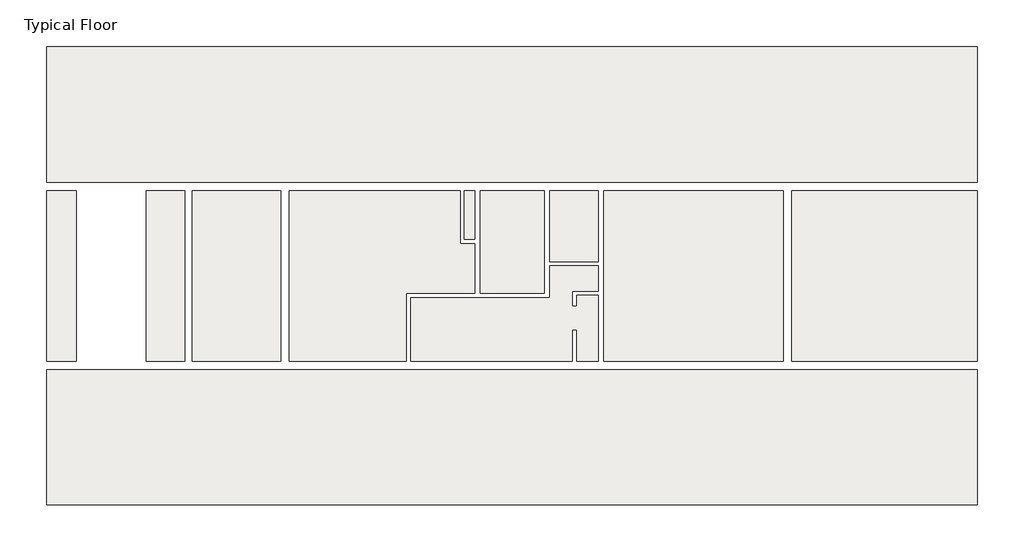
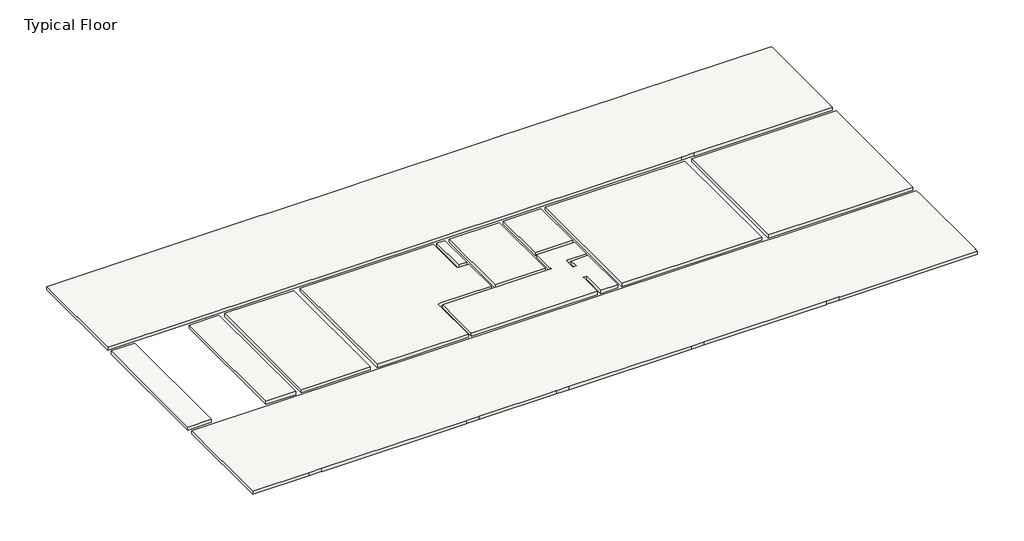
# One storey: 12 slabs.
"""IFC4 building model written with IfcOpenShell, lengths in millimetres."""

import ifcopenshell
import ifcopenshell.guid

model = None  # the IFC model being written
_history = None  # IfcOwnerHistory: only IFC2X3 demands one
_inside = {}  # id of a spatial element -> (the spatial element, [elements in it])
_under = {}  # id of a project, library or spatial element -> (it, [spatial elements below it])
_declared = {}  # id of a project -> (the project, [libraries it declares])
_typed = {}  # id of a type object -> (the type object, [elements of that type])
_made_of = {}  # id of a material, layer set ... -> (it, [elements and type objects made of it])


def new_model(schema):
    """Start an empty IFC model of exactly this schema.

    Asked for "IFC4X3", IfcOpenShell would pick the latest addendum, in which some entities
    have other attributes; the version numbers below select the first issue.
    IFC2X3 requires an IfcOwnerHistory on every rooted entity: one is made here for all.
    """
    global model, _history
    if schema == "IFC4X3":
        model = ifcopenshell.file(schema_version=(4, 3, 0, 0))
    else:
        model = ifcopenshell.file(schema=schema)
    _inside.clear()
    _under.clear()
    _declared.clear()
    _typed.clear()
    _made_of.clear()
    _history = None
    if model.schema == "IFC2X3":
        org = make("IfcOrganization", Name="unknown")
        user = make(
            "IfcPersonAndOrganization",
            ThePerson=make("IfcPerson", FamilyName="unknown"),
            TheOrganization=org,
        )
        app = make(
            "IfcApplication",
            ApplicationDeveloper=org,
            Version="unknown",
            ApplicationFullName="unknown",
            ApplicationIdentifier="unknown",
        )
        _history = make(
            "IfcOwnerHistory",
            OwningUser=user,
            OwningApplication=app,
            ChangeAction="ADDED",
            CreationDate=0,
        )
    return model


def make(cls, **values):
    """One entity of the class cls with the attributes given. An attribute that is None is left unset."""
    return model.create_entity(
        cls, **{name: value for name, value in values.items() if value is not None}
    )


def rooted(cls, **values):
    """An entity with a GlobalId (a new one), such as an element, a storey or a relation."""
    return make(cls, GlobalId=ifcopenshell.guid.new(), OwnerHistory=_history, **values)


def si_unit(unit_type, name, prefix=None):
    """IfcSIUnit, for example si_unit("LENGTHUNIT", "METRE", prefix="MILLI")."""
    return make("IfcSIUnit", UnitType=unit_type, Prefix=prefix, Name=name)


def assignment(units):
    """IfcUnitAssignment: the units of a project."""
    return None if units is None else make("IfcUnitAssignment", Units=units)


def point(xyz):
    """IfcCartesianPoint."""
    return None if xyz is None else make("IfcCartesianPoint", Coordinates=xyz)


def direction(xyz):
    """IfcDirection."""
    return None if xyz is None else make("IfcDirection", DirectionRatios=xyz)


def frame(location, z_axis=None, x_axis=None):
    """IfcAxis2Placement3D, a coordinate frame: its origin and axes. An axis left out is left unset."""
    return make(
        "IfcAxis2Placement3D",
        Location=point(location),
        Axis=direction(z_axis),
        RefDirection=direction(x_axis),
    )


def origin():
    """The frame at (0, 0, 0) with its axes left unset."""
    return frame((0.0, 0.0, 0.0))


def place(relative_to, where):
    """IfcLocalPlacement: puts the frame where relative to a parent placement (None: the world)."""
    return make(
        "IfcLocalPlacement", PlacementRelTo=relative_to, RelativePlacement=where
    )


def context(
    kind, dimensions, precision=None, world=None, true_north=None, identifier=None
):
    """IfcGeometricRepresentationContext, for example the 3D "Model" context."""
    return make(
        "IfcGeometricRepresentationContext",
        ContextIdentifier=identifier,
        ContextType=kind,
        CoordinateSpaceDimension=dimensions,
        Precision=precision,
        WorldCoordinateSystem=world,
        TrueNorth=true_north,
    )


def project(units=None, contexts=None):
    """IfcProject with its units and contexts."""
    return rooted(
        "IfcProject",
        Name="project",
        RepresentationContexts=contexts,
        UnitsInContext=assignment(units),
    )


def spatial(cls, under=None, at=None, **own):
    """A site, building, storey or space (cls), placed at a placement, below another one or the project."""
    s = rooted(cls, ObjectPlacement=at, **own)
    if under is not None:
        _under.setdefault(under.id(), (under, []))[1].append(s)
    return s


def polyline(points):
    """IfcPolyline through the points."""
    return make("IfcPolyline", Points=[point(p) for p in points])


def outline(outer, holes=None, kind="AREA"):
    """IfcArbitraryClosedProfileDef: a profile drawn as a closed curve; with holes, ...WithVoids."""
    if holes is None:
        return make("IfcArbitraryClosedProfileDef", ProfileType=kind, OuterCurve=outer)
    return make(
        "IfcArbitraryProfileDefWithVoids",
        ProfileType=kind,
        OuterCurve=outer,
        InnerCurves=holes,
    )


def extrude(swept, where, along, depth):
    """IfcExtrudedAreaSolid: the profile swept, set in the frame where, extruded along a direction by depth."""
    return make(
        "IfcExtrudedAreaSolid",
        SweptArea=swept,
        Position=where,
        ExtrudedDirection=direction(along),
        Depth=depth,
    )


def faces_of(points, faces, orient=None, outer=None):
    """IfcFace entities. A face is a list of loops; a loop is a list of indices into points, from 0.

    orient and outer hold one flag for each loop. By default every Orientation is true, the
    first loop of a face is its IfcFaceOuterBound and the others are IfcFaceBound.
    """
    made = []
    for i, loops in enumerate(faces):
        bounds = []
        for j, loop in enumerate(loops):
            is_outer = j == 0 if outer is None else outer[i][j]
            bounds.append(
                make(
                    "IfcFaceOuterBound" if is_outer else "IfcFaceBound",
                    Bound=make("IfcPolyLoop", Polygon=[points[k] for k in loop]),
                    Orientation=True if orient is None else orient[i][j],
                )
            )
        made.append(make("IfcFace", Bounds=bounds))
    return made


def faceted_brep(points, faces, orient=None, outer=None, voids=None):
    """IfcFacetedBrep: a solid bounded by flat faces; with voids (closed shells), ...WithVoids."""
    shared = [point(p) for p in points]
    hull = make("IfcClosedShell", CfsFaces=faces_of(shared, faces, orient, outer))
    if voids is None:
        return make("IfcFacetedBrep", Outer=hull)
    return make(
        "IfcFacetedBrepWithVoids",
        Outer=hull,
        Voids=[
            make(cls, CfsFaces=faces_of(shared, fs, o, b)) for cls, fs, o, b in voids
        ],
    )


def shape(context_of_items, identifier, shape_type, items):
    """IfcShapeRepresentation: the items that make up one representation, for example the "Body"."""
    return make(
        "IfcShapeRepresentation",
        ContextOfItems=context_of_items,
        RepresentationIdentifier=identifier,
        RepresentationType=shape_type,
        Items=items,
    )


def made_of(thing, what):
    """Note that an element or type object is made of a material, layer set ...; save() writes the relation."""
    if what is not None:
        _made_of.setdefault(what.id(), (what, []))[1].append(thing)
    return thing


def element(
    cls,
    number,
    at=None,
    inside=None,
    cuts=None,
    type_object=None,
    material=None,
    context=None,
    identifier="Body",
    shape_type=None,
    held_by="IfcProductDefinitionShape",
    body=None,
    shapes=None,
    **own,
):
    """One element of the class cls, such as IfcWall. Its Tag is "e" and its number.

    at: its placement. inside: the storey or other place that contains it. cuts: it is an
    opening in that element (IfcRelVoidsElement). A single representation is given by context,
    identifier, shape_type and body (its items); several are given by shapes. held_by: the class
    of the entity that holds the representations. save() writes the other relations.
    """
    e = rooted(cls, Tag="e%d" % number, ObjectPlacement=at, **own)
    if body is not None:
        shapes = [shape(context, identifier, shape_type, body)]
    if shapes is not None:
        e.Representation = make(held_by, Representations=shapes)
    if inside is not None:
        _inside.setdefault(inside.id(), (inside, []))[1].append(e)
    if cuts is not None:
        rooted(
            "IfcRelVoidsElement", RelatingBuildingElement=cuts, RelatedOpeningElement=e
        )
    if type_object is not None:
        _typed.setdefault(type_object.id(), (type_object, []))[1].append(e)
    return made_of(e, material)


def aggregate(whole, parts):
    """IfcRelAggregates: a whole, such as a stair, and the parts it consists of."""
    return rooted("IfcRelAggregates", RelatingObject=whole, RelatedObjects=parts)


def save(model, path):
    """Write the relations noted so far, then the file.

    IfcRelAggregates (storeys below a building ...), IfcRelContainedInSpatialStructure (elements
    in a storey), IfcRelDefinesByType, IfcRelAssociatesMaterial and IfcRelDeclares: one each for
    every whole, place, type object, material and project.
    """
    for whole, parts in _under.values():
        aggregate(whole, parts)
    for where, things in _inside.values():
        rooted(
            "IfcRelContainedInSpatialStructure",
            RelatedElements=things,
            RelatingStructure=where,
        )
    for kind, things in _typed.values():
        rooted("IfcRelDefinesByType", RelatedObjects=things, RelatingType=kind)
    for what, things in _made_of.values():
        rooted("IfcRelAssociatesMaterial", RelatedObjects=things, RelatingMaterial=what)
    for by, libraries in _declared.values():
        rooted("IfcRelDeclares", RelatingContext=by, RelatedDefinitions=libraries)
    model.write(path)


model = new_model("IFC4")

# Units and contexts
model_context = context("Model", 3, world=origin())
ifc_project = project(units=[si_unit("LENGTHUNIT", "METRE", prefix="MILLI")], contexts=[model_context])

# Site, building, storey
site = spatial("IfcSite", under=ifc_project)
building = spatial("IfcBuilding", under=site)
storey = spatial("IfcBuildingStorey", under=building, Name="Typical Floor", Elevation=3500.0)

# Slabs
placement = place(None, origin())
element("IfcSlab", 1, ObjectType="20", at=placement, inside=storey, context=model_context, shape_type="SweptSolid", body=[
    extrude(outline(polyline([(-28952.8929888, 3660.4573545), (-28952.8929888, -4379.553058), (-30362.89442, -4379.553058), (-30362.89442, 3660.4573545), (-28952.8929888, 3660.4573545)])), frame((0.0, 0.0, 3300.0), z_axis=(0.0, 0.0, 1.0), x_axis=(1.0, 0.0, 0.0)), (0.0, 0.0, 1.0), 200.0),
])
element("IfcSlab", 2, ObjectType="20", at=placement, inside=storey, context=model_context, shape_type="Brep", body=[
    faceted_brep([(-25647.8929888, 3660.4573545, 3300.0), (-23847.8929888, 3660.4573545, 3300.0), (-23847.8929888, -4379.553058, 3300.0), (-25647.8929888, -4379.553058, 3300.0), (-25647.8929888, 3660.4573545, 3500.0), (-25647.8929888, 2252.2215378, 3500.0), (-25647.8929888, 2002.2215378, 3500.0), (-25647.8929888, -4379.553058, 3500.0), (-23847.8929888, -4379.553058, 3500.0), (-23847.8929888, 3660.4573545, 3500.0)], [[[0, 1, 2, 3]], [[4, 5, 6, 7, 8, 9]], [[1, 0, 4, 9]], [[2, 1, 9, 8]], [[3, 2, 8, 7]], [[0, 3, 7, 6, 5, 4]]]),
])
element("IfcSlab", 3, ObjectType="20", at=placement, inside=storey, context=model_context, shape_type="SweptSolid", body=[
    extrude(outline(polyline([(-23497.8929888, 3660.4573545), (-19308.8564427, 3660.4573545), (-19308.8564427, -4379.553058), (-23497.8929888, -4379.553058), (-23497.8929888, 3660.4573545)])), frame((0.0, 0.0, 3300.0), z_axis=(0.0, 0.0, 1.0), x_axis=(1.0, 0.0, 0.0)), (0.0, 0.0, 1.0), 200.0),
])
element("IfcSlab", 4, ObjectType="20", at=placement, inside=storey, context=model_context, shape_type="Brep", body=[
    faceted_brep([(-26172.8897575, 10457.1426775, 3300.0), (-26172.8897575, 10462.1426775, 3300.0), (-17432.8798137, 10462.1426775, 3300.0), (-17432.8798137, 10457.1426775, 3300.0), (-16632.8798137, 10457.1426775, 3300.0), (-16632.8798137, 10462.1426775, 3300.0), (-11972.875695, 10462.1426775, 3300.0), (-11972.875695, 10457.1426775, 3300.0), (-11172.875695, 10457.1426775, 3300.0), (-11172.875695, 10462.1426775, 3300.0), (-3792.8676512, 10462.1426775, 3300.0), (-3792.8676512, 10460.462042, 3300.0), (-3392.8676512, 10460.462042, 3300.0), (-2992.8676512, 10460.462042, 3300.0), (-2992.8676512, 10462.1426775, 3300.0), (4387.1402675, 10462.1426775, 3300.0), (4387.1402675, 10460.462042, 3300.0), (5187.1402675, 10460.462042, 3300.0), (5187.1402675, 10462.1426775, 3300.0), (13547.1501363, 10462.1426775, 3300.0), (13547.1501363, 10460.462042, 3300.0), (13547.1501363, 10260.462042, 3300.0), (13552.1501363, 10260.462042, 3300.0), (13552.1501363, 4260.456417, 3300.0), (13547.1501363, 4260.456417, 3300.0), (13547.1501363, 4060.4573545, 3300.0), (13547.1501363, 4055.4573545, 3300.0), (5187.1402675, 4055.4573545, 3300.0), (5187.1402675, 4060.4573545, 3300.0), (4387.1402675, 4060.4573545, 3300.0), (4387.1402675, 4055.4573545, 3300.0), (-30362.89442, 4055.4573545, 3300.0), (-30362.89442, 4060.4573545, 3300.0), (-30362.89442, 10457.1426775, 3300.0), (-30362.89442, 10462.1426775, 3300.0), (-26972.8897575, 10462.1426775, 3300.0), (-26972.8897575, 10457.1426775, 3300.0), (-26172.8897575, 10462.1426775, 3500.0), (-26172.8897575, 10457.1426775, 3500.0), (-26972.8897575, 10457.1426775, 3500.0), (-26972.8897575, 10462.1426775, 3500.0), (-30362.89442, 10462.1426775, 3500.0), (-30362.89442, 4055.4573545, 3500.0), (4387.1402675, 4055.4573545, 3500.0), (4387.1402675, 4060.4573545, 3500.0), (5187.1402675, 4060.4573545, 3500.0), (5187.1402675, 4055.4573545, 3500.0), (13547.1501363, 4055.4573545, 3500.0), (13547.1501363, 4260.456417, 3500.0), (13552.1501363, 4260.456417, 3500.0), (13552.1501363, 10260.462042, 3500.0), (13547.1501363, 10260.462042, 3500.0), (13547.1501363, 10462.1426775, 3500.0), (5187.1402675, 10462.1426775, 3500.0), (5187.1402675, 10460.462042, 3500.0), (4387.1402675, 10460.462042, 3500.0), (4387.1402675, 10462.1426775, 3500.0), (-2992.8676512, 10462.1426775, 3500.0), (-2992.8676512, 10460.462042, 3500.0), (-3792.8676512, 10460.462042, 3500.0), (-3792.8676512, 10462.1426775, 3500.0), (-11172.875695, 10462.1426775, 3500.0), (-11172.875695, 10457.1426775, 3500.0), (-11972.875695, 10457.1426775, 3500.0), (-11972.875695, 10462.1426775, 3500.0), (-16632.8798137, 10462.1426775, 3500.0), (-16632.8798137, 10457.1426775, 3500.0), (-17432.8798137, 10457.1426775, 3500.0), (-17432.8798137, 10462.1426775, 3500.0)], [[[0, 1, 2, 3, 4, 5, 6, 7, 8, 9, 10, 11, 12, 13, 14, 15, 16, 17, 18, 19, 20, 21, 22, 23, 24, 25, 26, 27, 28, 29, 30, 31, 32, 33, 34, 35, 36]], [[37, 38, 39, 40, 41, 42, 43, 44, 45, 46, 47, 48, 49, 50, 51, 52, 53, 54, 55, 56, 57, 58, 59, 60, 61, 62, 63, 64, 65, 66, 67, 68]], [[22, 50, 49, 23]], [[46, 27, 26, 47]], [[30, 43, 42, 31]], [[9, 61, 60, 10]], [[5, 65, 64, 6]], [[1, 37, 68, 2]], [[40, 35, 34, 41]], [[18, 53, 52, 19]], [[14, 57, 56, 15]], [[0, 38, 37, 1]], [[38, 0, 36, 39]], [[39, 36, 35, 40]], [[4, 66, 65, 5]], [[66, 4, 3, 67]], [[67, 3, 2, 68]], [[8, 62, 61, 9]], [[62, 8, 7, 63]], [[63, 7, 6, 64]], [[28, 45, 44, 29]], [[45, 28, 27, 46]], [[29, 44, 43, 30]], [[13, 58, 57, 14]], [[58, 13, 12, 11, 59]], [[59, 11, 10, 60]], [[17, 54, 53, 18]], [[54, 17, 16, 55]], [[55, 16, 15, 56]], [[21, 51, 50, 22]], [[51, 21, 20, 19, 52]], [[48, 24, 23, 49]], [[24, 48, 47, 26, 25]], [[34, 33, 32, 31, 42, 41]]]),
])
element("IfcSlab", 5, ObjectType="20", at=placement, inside=storey, context=model_context, shape_type="Brep", body=[
    faceted_brep([(5187.1402675, -11159.5591018, 3300.0), (4387.1402675, -11159.5591018, 3300.0), (4387.1402675, -11164.5591018, 3300.0), (-2992.8676512, -11164.5591018, 3300.0), (-2992.8676512, -11159.5591018, 3300.0), (-3792.8676512, -11159.5591018, 3300.0), (-3792.8676512, -11164.5591018, 3300.0), (-11172.875695, -11164.5591018, 3300.0), (-11172.875695, -11159.5591018, 3300.0), (-11972.875695, -11159.5591018, 3300.0), (-11972.875695, -11164.5591018, 3300.0), (-16632.8798137, -11164.5591018, 3300.0), (-16632.8798137, -11159.5591018, 3300.0), (-17432.8798137, -11159.5591018, 3300.0), (-17432.8798137, -11164.5591018, 3300.0), (-26172.8897575, -11164.5591018, 3300.0), (-26172.8897575, -11159.5591018, 3300.0), (-26972.8897575, -11159.5591018, 3300.0), (-26972.8897575, -11164.5591018, 3300.0), (-30362.89442, -11164.5591018, 3300.0), (-30362.89442, -11159.5591018, 3300.0), (-30362.89442, -4779.553058, 3300.0), (-30362.89442, -4774.553058, 3300.0), (4387.1402675, -4774.553058, 3300.0), (4387.1402675, -4779.553058, 3300.0), (5187.1402675, -4779.553058, 3300.0), (5187.1402675, -4774.553058, 3300.0), (13547.1501363, -4774.553058, 3300.0), (13547.1501363, -4779.553058, 3300.0), (13547.1501363, -4979.5501205, 3300.0), (13552.10558, -4979.5501205, 3300.0), (13552.10558, -10959.5591018, 3300.0), (13547.1501363, -10959.5591018, 3300.0), (13547.1501363, -11159.5591018, 3300.0), (13547.1501363, -11164.5591018, 3300.0), (5187.1402675, -11164.5591018, 3300.0), (4387.1402675, -11159.5591018, 3500.0), (5187.1402675, -11159.5591018, 3500.0), (5187.1402675, -11164.5591018, 3500.0), (13547.1501363, -11164.5591018, 3500.0), (13547.1501363, -10959.5591018, 3500.0), (13552.10558, -10959.5591018, 3500.0), (13552.10558, -4979.5501205, 3500.0), (13547.1501363, -4979.5501205, 3500.0), (13547.1501363, -4774.553058, 3500.0), (5187.1402675, -4774.553058, 3500.0), (5187.1402675, -4779.553058, 3500.0), (4387.1402675, -4779.553058, 3500.0), (4387.1402675, -4774.553058, 3500.0), (-30362.89442, -4774.553058, 3500.0), (-30362.89442, -11164.5591018, 3500.0), (-26972.8897575, -11164.5591018, 3500.0), (-26972.8897575, -11159.5591018, 3500.0), (-26172.8897575, -11159.5591018, 3500.0), (-26172.8897575, -11164.5591018, 3500.0), (-17432.8798137, -11164.5591018, 3500.0), (-17432.8798137, -11159.5591018, 3500.0), (-16632.8798137, -11159.5591018, 3500.0), (-16632.8798137, -11164.5591018, 3500.0), (-11972.875695, -11164.5591018, 3500.0), (-11972.875695, -11159.5591018, 3500.0), (-11172.875695, -11159.5591018, 3500.0), (-11172.875695, -11164.5591018, 3500.0), (-3792.8676512, -11164.5591018, 3500.0), (-3792.8676512, -11159.5591018, 3500.0), (-2992.8676512, -11159.5591018, 3500.0), (-2992.8676512, -11164.5591018, 3500.0), (4387.1402675, -11164.5591018, 3500.0)], [[[0, 1, 2, 3, 4, 5, 6, 7, 8, 9, 10, 11, 12, 13, 14, 15, 16, 17, 18, 19, 20, 21, 22, 23, 24, 25, 26, 27, 28, 29, 30, 31, 32, 33, 34, 35]], [[36, 37, 38, 39, 40, 41, 42, 43, 44, 45, 46, 47, 48, 49, 50, 51, 52, 53, 54, 55, 56, 57, 58, 59, 60, 61, 62, 63, 64, 65, 66, 67]], [[30, 42, 41, 31]], [[2, 67, 66, 3]], [[6, 63, 62, 7]], [[10, 59, 58, 11]], [[14, 55, 54, 15]], [[38, 35, 34, 39]], [[18, 51, 50, 19]], [[26, 45, 44, 27]], [[48, 23, 22, 49]], [[0, 37, 36, 1]], [[37, 0, 35, 38]], [[1, 36, 67, 2]], [[4, 65, 64, 5]], [[65, 4, 3, 66]], [[5, 64, 63, 6]], [[8, 61, 60, 9]], [[61, 8, 7, 62]], [[9, 60, 59, 10]], [[12, 57, 56, 13]], [[57, 12, 11, 58]], [[13, 56, 55, 14]], [[16, 53, 52, 17]], [[53, 16, 15, 54]], [[17, 52, 51, 18]], [[25, 46, 45, 26]], [[46, 25, 24, 47]], [[47, 24, 23, 48]], [[29, 43, 42, 30]], [[43, 29, 28, 27, 44]], [[40, 32, 31, 41]], [[32, 40, 39, 34, 33]], [[22, 21, 20, 19, 50, 49]]]),
])
element("IfcSlab", 6, ObjectType="20", at=placement, inside=storey, context=model_context, shape_type="Brep", body=[
    faceted_brep([(13547.1501363, 3660.4573545, 3300.0), (13547.1501363, -4379.553058, 3300.0), (4787.1402675, -4379.553058, 3300.0), (4787.1402675, 3660.4573545, 3300.0), (13547.1501363, 3660.4573545, 3500.0), (5187.1402675, 3660.4573545, 3500.0), (4787.1402675, 3660.4573545, 3500.0), (4787.1402675, -4379.553058, 3500.0), (5187.1402675, -4379.553058, 3500.0), (13547.1501363, -4379.553058, 3500.0), (13547.1501363, -4179.5501205, 3500.0), (13547.1501363, 3460.456417, 3500.0)], [[[0, 1, 2, 3]], [[4, 5, 6, 7, 8, 9, 10, 11]], [[1, 0, 4, 11, 10, 9]], [[2, 1, 9, 8, 7]], [[3, 2, 7, 6]], [[0, 3, 6, 5, 4]]]),
])
element("IfcSlab", 7, ObjectType="20", at=placement, inside=storey, context=model_context, shape_type="SweptSolid", body=[
    extrude(outline(polyline([(4387.1402675, 3660.4573545), (4387.1402675, -4379.553058), (-4087.2434753, -4379.553058), (-4087.2434753, 3660.4573545), (4387.1402675, 3660.4573545)])), frame((0.0, 0.0, 3300.0), z_axis=(0.0, 0.0, 1.0), x_axis=(1.0, 0.0, 0.0)), (0.0, 0.0, 1.0), 200.0),
])
element("IfcSlab", 8, ObjectType="20", at=placement, inside=storey, context=model_context, shape_type="Brep", body=[
    faceted_brep([(-4337.2434753, 120.446942, 3300.0), (-4337.2434753, -1079.553058, 3300.0), (-5552.8714262, -1079.553058, 3300.0), (-5552.8714262, -1799.553058, 3300.0), (-5352.8714262, -1799.553058, 3300.0), (-5352.8714262, -1279.553058, 3300.0), (-4337.2434753, -1279.553058, 3300.0), (-4337.2434753, -4379.553058, 3300.0), (-5352.8714262, -4379.553058, 3300.0), (-5352.8714262, -2899.5501705, 3300.0), (-5552.8714262, -2899.5501705, 3300.0), (-5552.8714262, -4379.553058, 3300.0), (-13192.6687444, -4379.553058, 3300.0), (-13192.6687444, -1379.553058, 3300.0), (-6622.8724137, -1379.553058, 3300.0), (-6622.8724137, 120.446942, 3300.0), (-4337.2434753, 120.446942, 3500.0), (-6622.8724137, 120.446942, 3500.0), (-6622.8724137, -1179.553058, 3500.0), (-6622.8724137, -1379.553058, 3500.0), (-13192.6687444, -1379.553058, 3500.0), (-13192.6687444, -4379.553058, 3500.0), (-5552.8714262, -4379.553058, 3500.0), (-5552.8714262, -2899.5501705, 3500.0), (-5352.8714262, -2899.5501705, 3500.0), (-5352.8714262, -4379.553058, 3500.0), (-4337.2434753, -4379.553058, 3500.0), (-4337.2434753, -1279.553058, 3500.0), (-5352.8714262, -1279.553058, 3500.0), (-5352.8714262, -1799.553058, 3500.0), (-5552.8714262, -1799.553058, 3500.0), (-5552.8714262, -1279.553058, 3500.0), (-5552.8714262, -1079.553058, 3500.0), (-4337.2434753, -1079.553058, 3500.0)], [[[0, 1, 2, 3, 4, 5, 6, 7, 8, 9, 10, 11, 12, 13, 14, 15]], [[16, 17, 18, 19, 20, 21, 22, 23, 24, 25, 26, 27, 28, 29, 30, 31, 32, 33]], [[1, 0, 16, 33]], [[2, 1, 33, 32]], [[3, 2, 32, 31, 30]], [[4, 3, 30, 29]], [[5, 4, 29, 28]], [[6, 5, 28, 27]], [[7, 6, 27, 26]], [[8, 7, 26, 25]], [[9, 8, 25, 24]], [[10, 9, 24, 23]], [[11, 10, 23, 22]], [[12, 11, 22, 21]], [[13, 12, 21, 20]], [[14, 13, 20, 19]], [[15, 14, 19, 18, 17]], [[0, 15, 17, 16]]]),
])
element("IfcSlab", 9, ObjectType="20", at=placement, inside=storey, context=model_context, shape_type="SweptSolid", body=[
    extrude(outline(polyline([(-6872.8724137, 3660.4573545), (-6872.8724137, -1179.553058), (-9902.8742387, -1179.553058), (-9902.8742387, 3660.4573545), (-6872.8724137, 3660.4573545)])), frame((0.0, 0.0, 3300.0), z_axis=(0.0, 0.0, 1.0), x_axis=(1.0, 0.0, 0.0)), (0.0, 0.0, 1.0), 200.0),
])
element("IfcSlab", 10, ObjectType="20", at=placement, inside=storey, context=model_context, shape_type="SweptSolid", body=[
    extrude(outline(polyline([(-4337.2434753, 3660.4573545), (-4337.2434753, 320.446942), (-6622.8724137, 320.446942), (-6622.8724137, 3660.4573545), (-4337.2434753, 3660.4573545)])), frame((0.0, 0.0, 3300.0), z_axis=(0.0, 0.0, 1.0), x_axis=(1.0, 0.0, 0.0)), (0.0, 0.0, 1.0), 200.0),
])
element("IfcSlab", 11, ObjectType="20", at=placement, inside=storey, context=model_context, shape_type="SweptSolid", body=[
    extrude(outline(polyline([(-10152.8742387, 3660.4573545), (-10152.8742387, 1360.4573545), (-10647.8742387, 1360.4573545), (-10647.8742387, 3660.4573545), (-10152.8742387, 3660.4573545)])), frame((0.0, 0.0, 3300.0), z_axis=(0.0, 0.0, 1.0), x_axis=(1.0, 0.0, 0.0)), (0.0, 0.0, 1.0), 200.0),
])
element("IfcSlab", 12, ObjectType="20", at=placement, inside=storey, context=model_context, shape_type="Brep", body=[
    faceted_brep([(-13392.6687444, -4379.553058, 3300.0), (-18908.8564427, -4379.553058, 3300.0), (-18908.8564427, 3660.4573545, 3300.0), (-10847.8742387, 3660.4573545, 3300.0), (-10847.8742387, 1160.4573545, 3300.0), (-10152.8742387, 1160.4573545, 3300.0), (-10152.8742387, -1179.553058, 3300.0), (-13392.6687444, -1179.553058, 3300.0), (-18908.8564427, -4379.553058, 3500.0), (-13392.6687444, -4379.553058, 3500.0), (-13392.6687444, -1179.553058, 3500.0), (-13192.6687444, -1179.553058, 3500.0), (-10152.8742387, -1179.553058, 3500.0), (-10152.8742387, 1160.4573545, 3500.0), (-10847.8742387, 1160.4573545, 3500.0), (-10847.8742387, 1360.4573545, 3500.0), (-10847.8742387, 3660.4573545, 3500.0), (-18908.8564427, 3660.4573545, 3500.0)], [[[0, 1, 2, 3, 4, 5, 6, 7]], [[8, 9, 10, 11, 12, 13, 14, 15, 16, 17]], [[1, 0, 9, 8]], [[2, 1, 8, 17]], [[3, 2, 17, 16]], [[4, 3, 16, 15, 14]], [[5, 4, 14, 13]], [[6, 5, 13, 12]], [[7, 6, 12, 11, 10]], [[0, 7, 10, 9]]]),
])

save(model, "model.ifc")

# Revit data of these elements
# Type "20"
#   Function = 0
#   Layers, outside or top first: 20 cm "Concrete" (function 1)
# Element 1 (IfcSlab, "20")
#   Mark = "S1"
#   SOFiSTiK_AMG_Comments = ""
#   Height Offset From Level = 0 cm
#   built-in parameter 1001954 = 1
#   SOFiSTiK_AMG_Scheduled = yes
#   SOFiSTiK_AMG_Adjusted = yes
#   Phase Created = New Construction
#   Materials on its faces: "Concrete"
# Element 2 (IfcSlab, "20")
#   Mark = "S2"
#   SOFiSTiK_AMG_Comments = ""
#   built-in parameter 1001955 = 3.14159 (stored number, unit not read)
#   Height Offset From Level = 0 cm
#   built-in parameter 1001954 = 1
#   SOFiSTiK_AMG_Scheduled = yes
#   SOFiSTiK_AMG_Adjusted = yes
#   Phase Created = New Construction
#   Materials on its faces: "Concrete"
# Element 3 (IfcSlab, "20")
#   Mark = "S3"
#   SOFiSTiK_AMG_Comments = ""
#   built-in parameter 1001955 = 3.14159 (stored number, unit not read)
#   Height Offset From Level = 0 cm
#   built-in parameter 1001954 = 1
#   SOFiSTiK_AMG_Scheduled = yes
#   SOFiSTiK_AMG_Adjusted = yes
#   Phase Created = New Construction
#   Materials on its faces: "Concrete"
# Element 4 (IfcSlab, "20")
#   Mark = "S4"
#   SOFiSTiK_AMG_Comments = ""
#   Height Offset From Level = 0 cm
#   built-in parameter 1001954 = 1
#   SOFiSTiK_AMG_Scheduled = yes
#   SOFiSTiK_AMG_Adjusted = yes
#   Phase Created = New Construction
#   Materials on its faces: "Concrete"
# Element 5 (IfcSlab, "20")
#   Mark = "S5"
#   SOFiSTiK_AMG_Comments = ""
#   Height Offset From Level = 0 cm
#   built-in parameter 1001954 = 1
#   SOFiSTiK_AMG_Scheduled = yes
#   SOFiSTiK_AMG_Adjusted = yes
#   Phase Created = New Construction
#   Materials on its faces: "Concrete"
# Element 6 (IfcSlab, "20")
#   Mark = "S6"
#   SOFiSTiK_AMG_Comments = ""
#   Height Offset From Level = 0 cm
#   built-in parameter 1001954 = 1
#   SOFiSTiK_AMG_Scheduled = yes
#   SOFiSTiK_AMG_Adjusted = yes
#   Phase Created = New Construction
#   Materials on its faces: "Concrete"
# Element 7 (IfcSlab, "20")
#   Mark = "S7"
#   SOFiSTiK_AMG_Comments = ""
#   Height Offset From Level = 0 cm
#   built-in parameter 1001954 = 1
#   SOFiSTiK_AMG_Scheduled = yes
#   SOFiSTiK_AMG_Adjusted = yes
#   Phase Created = New Construction
#   Materials on its faces: "Concrete"
# Element 8 (IfcSlab, "20")
#   Mark = "S8"
#   SOFiSTiK_AMG_Comments = ""
#   Height Offset From Level = 0 cm
#   built-in parameter 1001954 = 1
#   SOFiSTiK_AMG_Scheduled = yes
#   SOFiSTiK_AMG_Adjusted = yes
#   Phase Created = New Construction
#   Materials on its faces: "Concrete"
# Element 9 (IfcSlab, "20")
#   Mark = "S9"
#   SOFiSTiK_AMG_Comments = ""
#   Height Offset From Level = 0 cm
#   built-in parameter 1001954 = 1
#   SOFiSTiK_AMG_Scheduled = yes
#   SOFiSTiK_AMG_Adjusted = yes
#   Phase Created = New Construction
#   Materials on its faces: "Concrete"
# Element 10 (IfcSlab, "20")
#   Mark = "S10"
#   SOFiSTiK_AMG_Comments = ""
#   Height Offset From Level = 0 cm
#   built-in parameter 1001954 = 1
#   SOFiSTiK_AMG_Scheduled = yes
#   SOFiSTiK_AMG_Adjusted = yes
#   Phase Created = New Construction
#   Materials on its faces: "Concrete"
# Element 11 (IfcSlab, "20")
#   Mark = "S11"
#   SOFiSTiK_AMG_Comments = ""
#   Height Offset From Level = 0 cm
#   built-in parameter 1001954 = 1
#   SOFiSTiK_AMG_Scheduled = yes
#   SOFiSTiK_AMG_Adjusted = yes
#   Phase Created = New Construction
#   Materials on its faces: "Concrete"
# Element 12 (IfcSlab, "20")
#   Mark = "S12"
#   SOFiSTiK_AMG_Comments = ""
#   Height Offset From Level = 0 cm
#   built-in parameter 1001954 = 1
#   SOFiSTiK_AMG_Scheduled = yes
#   SOFiSTiK_AMG_Adjusted = yes
#   Phase Created = New Construction
#   Materials on its faces: "Concrete"
# Materials
#   "Concrete": class "Concrete", colour RGB 192 192 192, transparency 0, Keynote = "01000", Description = "Cast-in-place concrete", Cost = 0
